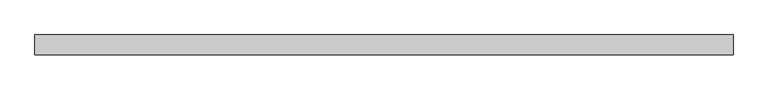
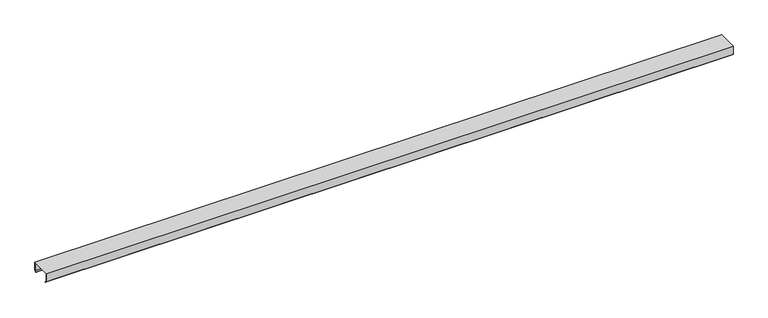
"""IFC4 building model written with IfcOpenShell, lengths in millimetres: proxy geometry, Generic Models 7:Generic Models 1:1:Generic Models 1:1 : Generic Models 7:Generic Models 1:337419:50 : Generic Models 7:Generic Models 1:1:Generic Models 1:1 : Generic Models 7:Generic Models 1:337419:306201."""

from ifc_helpers import new_model, si_unit, frame, origin, place, context, project, spatial, polyline, outline, extrude, source, transform, mapped, element, save


def generic_models_7a1d827f(model_context):
    return source(origin(), model_context, "Body", "SweptSolid", [
        extrude(outline(polyline([(-10.2195312, 0.0), (78.6804688, 0.0), (90.9255727, -14.5931466), (88.7974055, -16.3788909), (77.3850078, -2.778125), (-7.4414062, -2.778125), (-7.4414062, -200.421875), (77.3850078, -200.421875), (88.7974055, -186.821109), (90.9255727, -188.6068533), (78.6804688, -203.2), (-10.2195312, -203.2), (-10.2195312, 0.0)])), frame((573106.936724, -530645.4413842, 1299.2695313), z_axis=(1.0, -5.345279774360279e-12, 0.0), x_axis=(0.0, 0.0, -1.0)), (0.0, 0.0, 1.0), 7111.9999999),
    ])


if __name__ == "__main__":
    model = new_model("IFC4")
    model_context = context("Model", 3, world=origin())
    ifc_project = project(units=[si_unit("LENGTHUNIT", "METRE", prefix="MILLI")], contexts=[model_context])
    site = spatial("IfcSite", under=ifc_project)
    building = spatial("IfcBuilding", under=site)
    placement = place(None, origin())
    generic_models_shape = generic_models_7a1d827f(model_context)
    element("IfcBuildingElementProxy", 1, Name="Generic Models 7:Generic Models 1:1:Generic Models 1:1 : Generic Models 7:Generic Models 1:337419:50 : Generic Models 7:Generic Models 1:1:Generic Models 1:1 : Generic Models 7:Generic Models 1:337419:306201", ObjectType="Generic Models 7:Generic Models 1:1:Generic Models 1:1 : Generic Models 7:Generic Models 1:337419:50 : Generic Models 7:Generic Models 1:1:Generic Models 1:1 : Generic Models 7:Generic Models 1:337419:306201", at=placement, inside=building, context=model_context, shape_type="MappedRepresentation", body=[
        mapped(generic_models_shape, transform((0.0, 0.0, 0.0), x_axis=(1.0, 0.0, 0.0), y_axis=(0.0, 1.0, 0.0), z_axis=(0.0, 0.0, 1.0))),
    ])
    save(model, "model.ifc")

# Revit data of these elements
# Type "Generic Models 7:Generic Models 1:1:Generic Models 1:1 : Generic Models 7:Generic Models 1:337419:50 : Generic Models 7:Generic Models 1:1:Generic Models 1:1 : Generic Models 7:Generic Models 1:337419:306201"
#   NameOverride = "Generic Models 7:Generic Models 1:1:Generic Models 1:1 : Generic Models 7:Generic Models 1:337419:306201"
#   ObjectTypeOverride = "Generic Models 1:1 : Generic Models 7:Generic Models 1:337419"
#   Reference = "Generic Models 1"
#   Tag = "306201"
# Element 1 (IfcBuildingElementProxy, "Generic Models 7:Generic Models 1:1:Generic Models 1:1 : Generic Models 7:Generic Models 1:337419:50 : Generic Models 7:Generic Models 1:1:Generic Models 1:1 : Generic Models 7:Generic Models 1:337419:306201")
#   Materials on its faces: "CEE' SECTION (8.0x3.5C - SEE STRUCT. DWGS)"
# Materials
#   "CEE' SECTION (8.0x3.5C - SEE STRUCT. DWGS)": class "Unassigned", colour RGB 210 209 208, transparency 0, Keynote = "M05121300.02", Cost = 0
